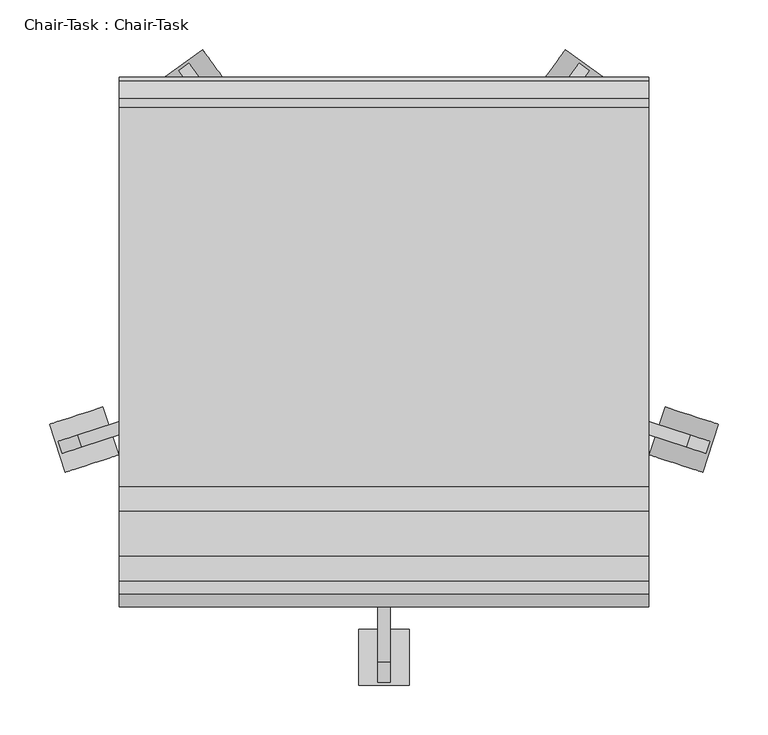
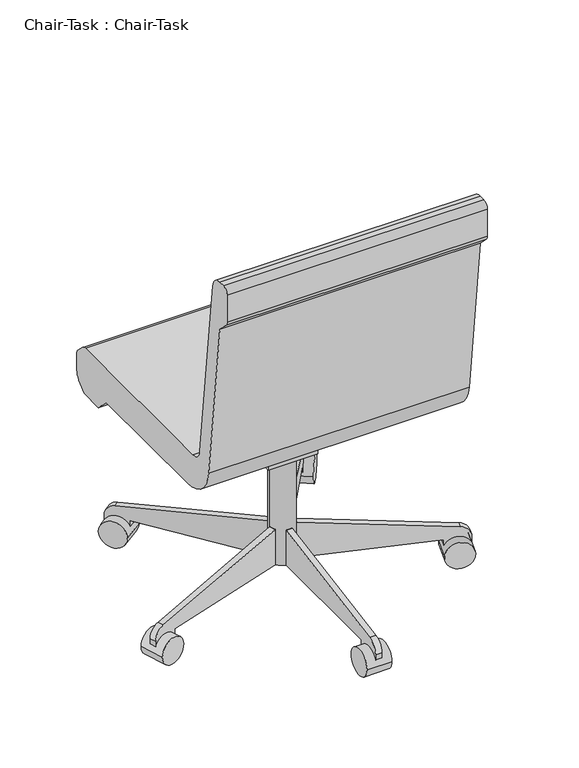
"""IFC4 building model written with IfcOpenShell, lengths in millimetres: furniture geometry, Chair-Task : Chair-Task."""

from ifc_helpers import new_model, si_unit, point, frame, frame_2d, origin, place, context, project, spatial, polyline, circle_curve, trimmed, segment, composite_curve, outline, extrude, source, transform, mapped, element, save


def chair_task_chair_task_e9ee4668(model_context):
    return source(origin(), model_context, "Body", "SweptSolid", [
        extrude(outline(composite_curve([segment(trimmed(circle_curve(frame_2d((0.0, -28.2002728)), 28.2002727), [point((0.0, -56.4005455))], [point((0.0, 0.0))], False, "CARTESIAN"), True, "CONTINUOUS"), segment(trimmed(circle_curve(frame_2d((0.0, -28.2002728)), 28.2002727), [point((0.0, 0.0))], [point((0.0, -56.4005455))], False, "CARTESIAN"), True, "CONTINUOUS")], self_intersect=False)), frame((461.9222851, -112.0381931, 28.1835944), z_axis=(0.30901699437494234, 0.9510565162951552, 0.0), x_axis=(0.0, 0.0, 1.0)), (0.0, 0.0, 1.0), 50.8),
        extrude(outline(composite_curve([segment(polyline([(292.1, 0.0), (292.1, 25.4), (342.9, 25.4), (342.9, 1.096947)]), True, "CONTINUOUS"), segment(trimmed(circle_curve(frame_2d((317.5, 1.096947)), 25.4), [point((342.9, 1.096947))], [point((321.9106636, -23.9171699))], False, "CARTESIAN"), True, "CONTINUOUS"), segment(polyline([(321.9106636, -23.9171699), (25.4, -76.2), (0.0, -76.2), (0.0, 0.0), (292.1, 0.0)]), True, "CONTINUOUS")], self_intersect=False)), frame((139.0285618, 12.9066928, 53.5835944), z_axis=(0.30901699437494234, 0.9510565162951552, 0.0), x_axis=(0.9510565162951552, -0.30901699437494234, 0.0)), (0.0, 0.0, 1.0), 12.7),
        extrude(outline(composite_curve([segment(trimmed(circle_curve(frame_2d((0.0, -28.2002727)), 28.2002727), [point((0.0, -56.4005454))], [point((0.0, 0.0))], False, "CARTESIAN"), True, "CONTINUOUS"), segment(trimmed(circle_curve(frame_2d((0.0, -28.2002727)), 28.2002727), [point((0.0, 0.0))], [point((0.0, -56.4005454))], False, "CARTESIAN"), True, "CONTINUOUS")], self_intersect=False)), frame((364.7373733, 283.6935518, 28.1835944), z_axis=(-0.8090169943749497, 0.58778525229247, 0.0), x_axis=(0.0, 0.0, 1.0)), (0.0, 0.0, 1.0), 50.8),
        extrude(outline(composite_curve([segment(polyline([(292.1, 0.0), (292.1, 25.4), (342.9, 25.4), (342.9, 1.096947)]), True, "CONTINUOUS"), segment(trimmed(circle_curve(frame_2d((317.5, 1.096947)), 25.4), [point((342.9, 1.096947))], [point((321.9106637, -23.9171699))], False, "CARTESIAN"), True, "CONTINUOUS"), segment(polyline([(321.9106637, -23.9171699), (25.3999999, -76.2), (0.0, -76.2), (0.0, 0.0), (292.1, 0.0)]), True, "CONTINUOUS")], self_intersect=False)), frame((146.1280776, 15.2134653, 53.5835944), z_axis=(-0.8090169943749498, 0.58778525229247, 0.0), x_axis=(0.58778525229247, 0.8090169943749498, 0.0)), (0.0, 0.0, 1.0), 12.7),
        extrude(outline(composite_curve([segment(trimmed(circle_curve(frame_2d((0.0, -28.2002727)), 28.2002727), [point((0.0, -56.4005454))], [point((0.0, 0.0))], False, "CARTESIAN"), True, "CONTINUOUS"), segment(trimmed(circle_curve(frame_2d((0.0, -28.2002727)), 28.2002727), [point((0.0, 0.0))], [point((0.0, -56.4005454))], False, "CARTESIAN"), True, "CONTINUOUS")], self_intersect=False)), frame((-82.755734, 283.6935518, 28.1835944), z_axis=(0.8090169943749459, 0.5877852522924751, 0.0), x_axis=(0.0, 0.0, -1.0)), (0.0, 0.0, 1.0), 50.8),
        extrude(outline(composite_curve([segment(polyline([(-292.1, 0.0), (0.0, 0.0), (0.0, -76.2), (-25.4, -76.2), (-321.9106637, -23.9171699)]), True, "CONTINUOUS"), segment(trimmed(circle_curve(frame_2d((-317.5, 1.096947)), 25.4), [point((-321.9106637, -23.9171699))], [point((-342.9000001, 1.096947))], False, "CARTESIAN"), True, "CONTINUOUS"), segment(polyline([(-342.9000001, 1.096947), (-342.9000001, 25.4), (-292.1, 25.4), (-292.1, 0.0)]), True, "CONTINUOUS")], self_intersect=False)), frame((135.8535618, 15.2134653, 53.5835944), z_axis=(0.8090169943749459, 0.5877852522924752, 0.0), x_axis=(0.5877852522924752, -0.8090169943749459, 0.0)), (0.0, 0.0, 1.0), 12.7),
        extrude(outline(composite_curve([segment(trimmed(circle_curve(frame_2d((0.0, -28.2002727)), 28.2002727), [point((0.0, -56.4005454))], [point((0.0, 0.0))], False, "CARTESIAN"), True, "CONTINUOUS"), segment(trimmed(circle_curve(frame_2d((0.0, -28.2002727)), 28.2002727), [point((0.0, 0.0))], [point((0.0, -56.4005454))], False, "CARTESIAN"), True, "CONTINUOUS")], self_intersect=False)), frame((-179.9406457, -112.0381931, 28.1835944), z_axis=(-0.30901699437494856, 0.9510565162951532, 0.0), x_axis=(0.0, 0.0, -1.0)), (0.0, 0.0, 1.0), 50.8),
        extrude(outline(composite_curve([segment(polyline([(-292.1, 0.0), (0.0, 0.0), (0.0, -76.2), (-25.4, -76.2), (-321.9106637, -23.9171699)]), True, "CONTINUOUS"), segment(trimmed(circle_curve(frame_2d((-317.5, 1.096947)), 25.4), [point((-321.9106637, -23.9171699))], [point((-342.9000001, 1.096947))], False, "CARTESIAN"), True, "CONTINUOUS"), segment(polyline([(-342.9000001, 1.096947), (-342.9000001, 25.4), (-292.1, 25.4), (-292.1, 0.0)]), True, "CONTINUOUS")], self_intersect=False)), frame((142.9530776, 12.9066928, 53.5835944), z_axis=(-0.30901699437494856, 0.9510565162951532, 0.0), x_axis=(0.9510565162951532, 0.30901699437494856, 0.0)), (0.0, 0.0, 1.0), 12.7),
        extrude(outline(composite_curve([segment(trimmed(circle_curve(frame_2d((-298.5540984, 28.1835944)), 28.2002727), [point((-270.3538256, 28.1835944))], [point((-326.7543711, 28.1835944))], False, "CARTESIAN"), True, "CONTINUOUS"), segment(trimmed(circle_curve(frame_2d((-298.5540984, 28.1835944)), 28.2002727), [point((-326.7543711, 28.1835944))], [point((-270.3538256, 28.1835944))], False, "CARTESIAN"), True, "CONTINUOUS")], self_intersect=False)), frame((115.5908197, 0.0, 0.0), z_axis=(1.0, 0.0, 0.0), x_axis=(0.0, 1.0, 0.0)), (0.0, 0.0, 1.0), 50.8),
        extrude(outline(composite_curve([segment(polyline([(-273.1540984, 53.5835944), (-273.1540984, 28.1835944), (-323.9540984, 28.1835944), (-323.9540984, 52.4866474)]), True, "CONTINUOUS"), segment(trimmed(circle_curve(frame_2d((-298.5540984, 52.4866474)), 25.4), [point((-323.9540984, 52.4866474))], [point((-302.9647621, 77.5007643))], False, "CARTESIAN"), True, "CONTINUOUS"), segment(polyline([(-302.9647621, 77.5007643), (-6.4540984, 129.7835944), (18.9459016, 129.7835944), (18.9459016, 53.5835944), (-273.1540984, 53.5835944)]), True, "CONTINUOUS")], self_intersect=False)), frame((134.6408197, 0.0, 0.0), z_axis=(1.0, 0.0, 0.0), x_axis=(0.0, 1.0, 0.0)), (0.0, 0.0, 1.0), 12.7),
        extrude(outline(composite_curve([segment(trimmed(circle_curve(frame_2d((140.9908197, 18.9459016)), 25.4), [point((115.5908197, 18.9459016))], [point((166.3908197, 18.9459016))], False, "CARTESIAN"), True, "CONTINUOUS"), segment(trimmed(circle_curve(frame_2d((140.9908197, 18.9459016)), 25.4), [point((166.3908197, 18.9459016))], [point((115.5908197, 18.9459016))], False, "CARTESIAN"), True, "CONTINUOUS")], self_intersect=False)), frame((0.0, 0.0, 53.5835944), z_axis=(0.0, 0.0, 1.0), x_axis=(1.0, 0.0, 0.0)), (0.0, 0.0, 1.0), 330.5914056),
        extrude(outline(polyline([(69.7459016, 383.7835944), (69.7459016, 371.0835944), (18.9459016, 283.0954134), (-19.1540984, 283.0954134), (-19.1540984, 383.7835944), (69.7459016, 383.7835944)])), frame((90.1908197, 0.0, 0.0), z_axis=(1.0, 0.0, 0.0), x_axis=(0.0, 1.0, 0.0)), (0.0, 0.0, 1.0), 101.6),
        extrude(outline(composite_curve([segment(polyline([(-126.2050455, 457.2), (255.0102301, 457.2)]), True, "CONTINUOUS"), segment(trimmed(circle_curve(frame_2d((255.0102301, 444.5)), 12.7), [point((255.0102301, 457.2))], [point((263.9604301, 453.510212))], False, "CARTESIAN"), True, "CONTINUOUS"), segment(polyline([(263.9604301, 453.510212), (281.8961016, 435.6939999)]), True, "CONTINUOUS"), segment(trimmed(circle_curve(frame_2d((272.9459016, 426.6837879)), 12.7), [point((281.8961016, 435.6939999))], [point((285.6459016, 426.6837879))], False, "CARTESIAN"), True, "CONTINUOUS"), segment(polyline([(285.6459016, 426.6837879), (285.6459016, 391.6405184)]), True, "CONTINUOUS"), segment(trimmed(circle_curve(frame_2d((260.2459016, 391.6405184)), 25.4), [point((285.6459016, 391.6405184))], [point((278.2663256, 373.7401184))], False, "CARTESIAN"), True, "CONTINUOUS"), segment(polyline([(278.2663256, 373.7401184), (260.2470284, 355.6), (209.4470284, 355.6), (181.0744602, 383.7835944), (-107.1089978, 383.7835944)]), True, "CONTINUOUS"), segment(trimmed(circle_curve(frame_2d((-107.1089978, 459.9835944)), 76.2), [point((-107.1089978, 383.7835944))], [point((-182.7870738, 451.0802913))], False, "CARTESIAN"), True, "CONTINUOUS"), segment(polyline([(-182.7870738, 451.0802913), (-222.3540984, 787.4), (-244.0343545, 809.0802561)]), True, "CONTINUOUS"), segment(trimmed(circle_curve(frame_2d((-235.0540984, 818.0605122)), 12.7), [point((-244.0343545, 809.0802561))], [point((-247.7540984, 818.0605122))], False, "CARTESIAN"), True, "CONTINUOUS"), segment(polyline([(-247.7540984, 818.0605122), (-247.7540984, 876.3)]), True, "CONTINUOUS"), segment(trimmed(circle_curve(frame_2d((-235.0540984, 876.3)), 12.7), [point((-247.7540984, 876.3))], [point((-235.0540984, 889.0))], False, "CARTESIAN"), True, "CONTINUOUS"), segment(polyline([(-235.0540984, 889.0), (-222.1789239, 889.0)]), True, "CONTINUOUS"), segment(trimmed(circle_curve(frame_2d((-222.1789239, 863.6)), 25.4), [point((-222.1789239, 889.0))], [point((-196.9528985, 866.5677677))], False, "CARTESIAN"), True, "CONTINUOUS"), segment(polyline([(-196.9528985, 866.5677677), (-151.4310708, 479.6322323)]), True, "CONTINUOUS"), segment(trimmed(circle_curve(frame_2d((-126.2050455, 482.6)), 25.4), [point((-151.4310708, 479.6322323))], [point((-126.2050455, 457.2))], True, "CARTESIAN"), True, "CONTINUOUS")], self_intersect=False)), frame((-125.7091803, 0.0, 0.0), z_axis=(1.0, 0.0, 0.0), x_axis=(0.0, 1.0, 0.0)), (0.0, 0.0, 1.0), 533.4),
    ])


if __name__ == "__main__":
    model = new_model("IFC4")
    model_context = context("Model", 3, world=origin())
    ifc_project = project(units=[si_unit("LENGTHUNIT", "METRE", prefix="MILLI")], contexts=[model_context])
    site = spatial("IfcSite", under=ifc_project)
    building = spatial("IfcBuilding", under=site)
    placement = place(None, origin())
    chair_task_chair_task_shape = chair_task_chair_task_e9ee4668(model_context)
    element("IfcFurniture", 1, ObjectType="Chair-Task : Chair-Task", at=placement, inside=building, context=model_context, shape_type="MappedRepresentation", body=[
        mapped(chair_task_chair_task_shape, transform((0.0, 0.0, 0.0), x_axis=(1.0, 0.0, 0.0), y_axis=(0.0, 1.0, 0.0), z_axis=(0.0, 0.0, 1.0))),
    ])
    save(model, "model.ifc")

# Revit data of these elements
# Type "Chair-Task : Chair-Task"
#   Model = "CHTSK-895"
#   Manufacturer = "Furniture Concepts"
#   Type Mark = "CH-4"
#   Assembly Code = "E2020200"
#   Cost = 895
#   Base Material = Plastic, Opaque Black
#   Caster Material = Plastic, Opaque Black
#   Seat/Back Material = Leather - Matte (Tan)
#   Default Elevation = 0
# Element 1 (IfcFurniture, "Chair-Task : Chair-Task")
#   Materials on its faces: "Plastic, Opaque Black", "Leather - Matte (Tan)"
# Materials
#   "Plastic, Opaque Black": class "Plastic", colour RGB 0 0 0, transparency 0, Description = "Plastic, generic, opaque black", Cost = 0
#   "Leather - Matte (Tan)": class "Generic", colour RGB 162 130 69, transparency 0, Cost = 0
